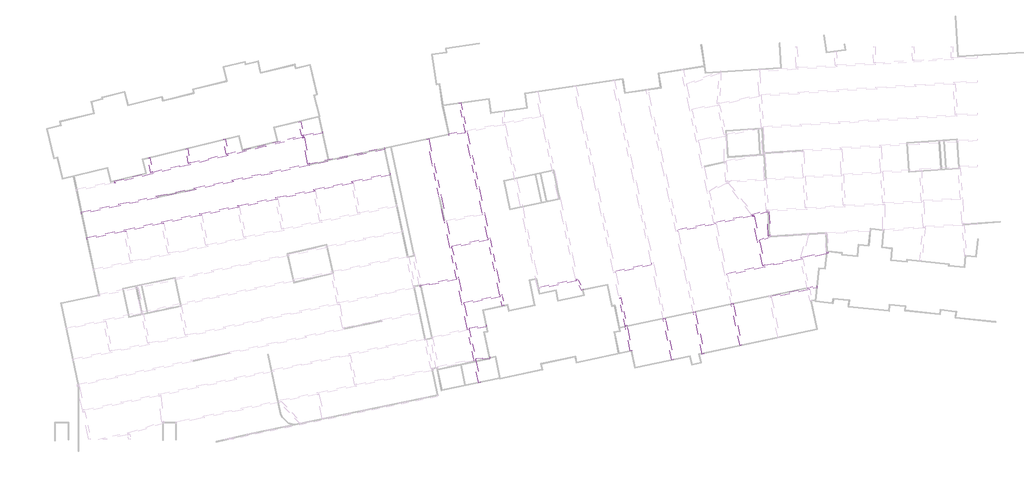
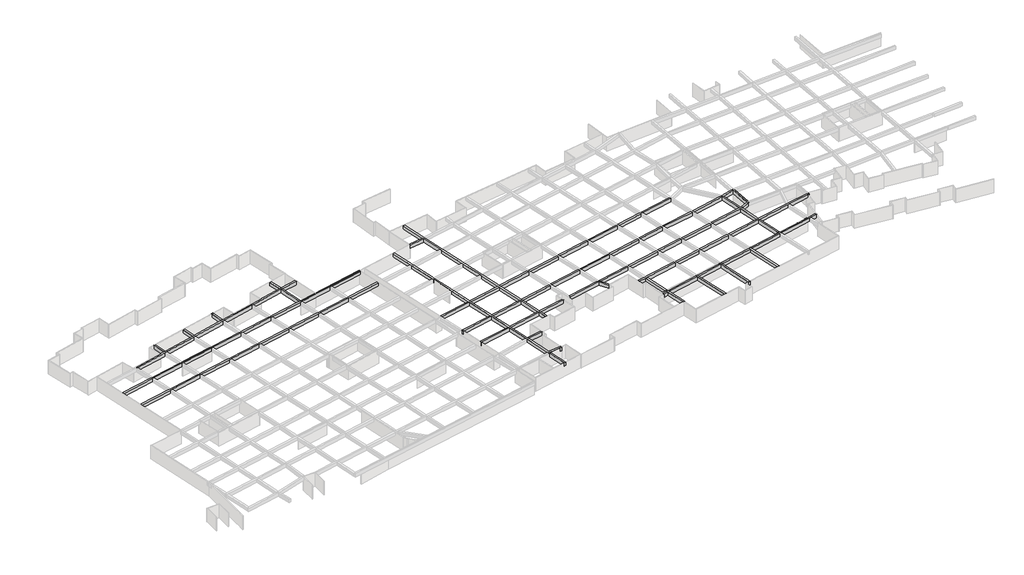
# One storey, part 9 of 14: 33 beams.
"""IFC4 building model written with IfcOpenShell, lengths in millimetres."""

from ifc_helpers import new_model, si_unit, frame, origin, place, context, project, spatial, polyline, outline, extrude, faceted_brep, element, save

model = new_model("IFC4")

# Units and contexts
model_context = context("Model", 3, world=origin())
ifc_project = project(units=[si_unit("LENGTHUNIT", "METRE", prefix="MILLI")], contexts=[model_context])

# Site, building, storey
site = spatial("IfcSite", under=ifc_project)
building = spatial("IfcBuilding", under=site)
storey = spatial("IfcBuildingStorey", under=building, Name="户型图", Elevation=0.0)

# Beams
placement = place(None, origin())
element("IfcBeam", 1, ObjectType="混凝土 - 矩形梁 : KL_beam", at=placement, inside=storey, context=model_context, shape_type="Brep", body=[
    faceted_brep([(-288393.3904984, -144066.4161825, 3300.0), (-303839.5822954, -147811.5548627, 3300.0), (-304228.7284594, -147905.9086277, 3300.0), (-311610.250183, -149695.6586768, 3300.0), (-311999.3963469, -149790.0124418, 3300.0), (-319359.3633104, -151574.5362469, 3300.0), (-319748.5094743, -151668.8900119, 3300.0), (-327267.044724, -153491.8608485, 3300.0), (-327178.3172304, -153881.9374755, 3300.0), (-326986.6349567, -153835.4615086, 3300.0), (-319668.5820962, -152061.1003462, 3300.0), (-319279.6883606, -151966.8077859, 3300.0), (-311919.2779813, -150182.1764686, 3300.0), (-311530.3946325, -150087.8864267, 3300.0), (-304148.8010812, -148298.1189621, 3300.0), (-303759.9073457, -148203.8264018, 3300.0), (-296335.6153384, -146403.7061174, 3300.0), (-295946.7216029, -146309.4135571, 3300.0), (-288504.0259967, -144504.8310706, 3300.0), (-288304.6630048, -144456.4928095, 3300.0), (-327178.3172304, -153881.9374755, 2500.0), (-326986.6349567, -153835.4615086, 2500.0), (-319668.5820962, -152061.1003462, 2500.0), (-319279.6883606, -151966.8077859, 2500.0), (-311919.2779813, -150182.1764686, 2500.0), (-311530.3946325, -150087.8864267, 2500.0), (-304148.8010812, -148298.1189621, 2500.0), (-303759.9073457, -148203.8264018, 2500.0), (-296335.6153384, -146403.7061174, 2500.0), (-295946.7216029, -146309.4135571, 2500.0), (-288504.0259967, -144504.8310706, 2500.0), (-288304.6630048, -144456.4928095, 2500.0), (-327267.044724, -153491.8608485, 2500.0), (-319748.5094743, -151668.8900119, 2500.0), (-319359.3633104, -151574.5362469, 2500.0), (-311999.3963469, -149790.0124418, 2500.0), (-311610.250183, -149695.6586768, 2500.0), (-304228.7284594, -147905.9086277, 2500.0), (-303839.5822954, -147811.5548627, 2500.0), (-288393.3904984, -144066.4161825, 2500.0)], [[[0, 1, 2, 3, 4, 5, 6, 7, 8, 9, 10, 11, 12, 13, 14, 15, 16, 17, 18, 19]], [[19, 18, 17, 16, 15, 14, 13, 12, 11, 10, 9, 8, 20, 21, 22, 23, 24, 25, 26, 27, 28, 29, 30, 31]], [[31, 30, 29, 28, 27, 26, 25, 24, 23, 22, 21, 20, 32, 33, 34, 35, 36, 37, 38, 39]], [[7, 6, 5, 4, 3, 2, 1, 0, 39, 38, 37, 36, 35, 34, 33, 32]], [[7, 32, 20, 8]], [[0, 19, 31, 39]]]),
])
element("IfcBeam", 2, ObjectType="混凝土 - 矩形梁 : KL_beam", at=placement, inside=storey, context=model_context, shape_type="Brep", body=[
    faceted_brep([(-284402.4891232, -143218.1239082, 3300.0), (-284319.3244469, -143609.3829485, 3300.0), (-284319.3244469, -143609.3829485, 2500.0), (-284402.4891232, -143218.1239082, 2500.0), (-288200.5117757, -144025.4185444, 3300.0), (-288393.3904984, -144066.4161825, 3300.0), (-288304.6630048, -144456.4928095, 3300.0), (-288113.8961147, -144415.9440553, 3300.0), (-288304.6630048, -144456.4928095, 2500.0), (-288113.8961147, -144415.9440553, 2500.0), (-288393.3904984, -144066.4161825, 2500.0), (-288200.5117757, -144025.4185444, 2500.0)], [[[0, 1, 2, 3]], [[1, 0, 4, 5, 6, 7]], [[2, 1, 7, 6, 8, 9]], [[3, 2, 9, 8, 10, 11]], [[0, 3, 11, 10, 5, 4]], [[5, 10, 8, 6]]]),
])
element("IfcBeam", 3, ObjectType="混凝土 - 矩形梁 : KL_beam", at=placement, inside=storey, context=model_context, shape_type="SweptSolid", body=[
    extrude(outline(polyline([(-289274.6055614, -141296.103949), (-288885.8925062, -141201.7526868), (-288200.5117757, -144025.4185444), (-288393.3904984, -144066.4161825), (-288590.5706614, -144114.2251872), (-289274.6055614, -141296.103949)])), frame((0.0, 0.0, 2500.0), z_axis=(0.0, 0.0, 1.0), x_axis=(1.0, 0.0, 0.0)), (0.0, 0.0, 1.0), 800.0),
])
element("IfcBeam", 4, ObjectType="混凝土 - 矩形梁 : KL_beam", at=placement, inside=storey, context=model_context, shape_type="SweptSolid", body=[
    extrude(outline(polyline([(-304823.3719195, -144846.7332269), (-304430.7210461, -144770.4096288), (-303839.5822954, -147811.5548627), (-304228.7284594, -147905.9086277), (-304823.3719195, -144846.7332269)])), frame((0.0, 0.0, 2500.0), z_axis=(0.0, 0.0, 1.0), x_axis=(1.0, 0.0, 0.0)), (0.0, 0.0, 1.0), 800.0),
])
element("IfcBeam", 5, ObjectType="混凝土 - 矩形梁 : KL_beam", at=placement, inside=storey, context=model_context, shape_type="SweptSolid", body=[
    extrude(outline(polyline([(-312574.5677396, -146831.0121441), (-312181.9168662, -146754.6885459), (-311610.250183, -149695.6586768), (-311999.3963469, -149790.0124418), (-312574.5677396, -146831.0121441)])), frame((0.0, 0.0, 2500.0), z_axis=(0.0, 0.0, 1.0), x_axis=(1.0, 0.0, 0.0)), (0.0, 0.0, 1.0), 800.0),
])
element("IfcBeam", 6, ObjectType="混凝土 - 矩形梁 : KL_beam", at=placement, inside=storey, context=model_context, shape_type="SweptSolid", body=[
    extrude(outline(polyline([(-320323.3003914, -148711.8470911), (-319930.649518, -148635.523493), (-319359.3633104, -151574.5362469), (-319748.5094743, -151668.8900119), (-320323.3003914, -148711.8470911)])), frame((0.0, 0.0, 2500.0), z_axis=(0.0, 0.0, 1.0), x_axis=(1.0, 0.0, 0.0)), (0.0, 0.0, 1.0), 800.0),
])
element("IfcBeam", 7, ObjectType="混凝土 - 矩形梁 : KL_beam", at=placement, inside=storey, context=model_context, shape_type="Brep", body=[
    faceted_brep([(-271576.7058607, -146561.7487568, 3300.0), (-271493.5411843, -146953.0077971, 3300.0), (-271493.5411843, -146953.0077971, 2500.0), (-271576.7058607, -146561.7487568, 2500.0), (-334091.0971712, -159849.5928286, 3300.0), (-334091.0971712, -159849.5928286, 2500.0), (-334007.9324948, -160240.8518689, 2500.0), (-334007.9324948, -160240.8518689, 3300.0), (-287020.5801813, -149844.4455812, 3300.0), (-287411.8616009, -149927.6150144, 3300.0), (-294841.9553377, -151506.930192, 3300.0), (-295233.214378, -151590.0948684, 3300.0), (-302702.6619422, -153177.7749602, 3300.0), (-303093.9209824, -153260.9396365, 3300.0), (-310515.8719459, -154838.5240142, 3300.0), (-310907.1311647, -154921.6887284, 3300.0), (-318316.8363826, -156496.6701926, 3300.0), (-318708.0954229, -156579.8348689, 3300.0), (-326070.6576793, -158144.7957872, 3300.0), (-326461.9167196, -158227.9604635, 3300.0), (-326378.7520433, -158619.2195038, 3300.0), (-325987.493003, -158536.0548275, 3300.0), (-318624.9307466, -156971.0939092, 3300.0), (-318233.6717063, -156887.9292328, 3300.0), (-310823.5927811, -155312.8683348, 3300.0), (-310432.3335623, -155229.7036205, 3300.0), (-303010.7563061, -153652.1986768, 3300.0), (-302619.4972658, -153569.0340005, 3300.0), (-295150.0497017, -151981.3539087, 3300.0), (-294758.7906614, -151898.1892323, 3300.0), (-287331.8776756, -150319.5501442, 3300.0), (-286940.6186353, -150236.3854679, 3300.0), (-279504.6810453, -148655.828141, 3300.0), (-279113.422005, -148572.6634647, 3300.0), (-326378.7520433, -158619.2195038, 2500.0), (-325987.493003, -158536.0548275, 2500.0), (-318624.9307466, -156971.0939092, 2500.0), (-318233.6717063, -156887.9292328, 2500.0), (-310823.5927811, -155312.8683348, 2500.0), (-310432.3335623, -155229.7036205, 2500.0), (-303010.7563061, -153652.1986768, 2500.0), (-302619.4972658, -153569.0340005, 2500.0), (-295150.0497017, -151981.3539087, 2500.0), (-294758.7906614, -151898.1892323, 2500.0), (-287331.8776756, -150319.5501442, 2500.0), (-286940.6186353, -150236.3854679, 2500.0), (-279504.6810453, -148655.828141, 2500.0), (-279113.422005, -148572.6634647, 2500.0), (-326461.9167196, -158227.9604635, 2500.0), (-326070.6576793, -158144.7957872, 2500.0), (-318708.0954229, -156579.8348689, 2500.0), (-318316.8363826, -156496.6701926, 2500.0), (-310907.1311647, -154921.6887284, 2500.0), (-310515.8719459, -154838.5240142, 2500.0), (-303093.9209824, -153260.9396365, 2500.0), (-302702.6619422, -153177.7749602, 2500.0), (-295233.214378, -151590.0948684, 2500.0), (-294841.9553377, -151506.930192, 2500.0), (-287411.8616009, -149927.6150144, 2500.0), (-287020.5801813, -149844.4455812, 2500.0)], [[[0, 1, 2, 3]], [[4, 5, 6, 7]], [[1, 0, 8, 9, 10, 11, 12, 13, 14, 15, 16, 17, 18, 19, 4, 7, 20, 21, 22, 23, 24, 25, 26, 27, 28, 29, 30, 31, 32, 33]], [[2, 1, 33, 32, 31, 30, 29, 28, 27, 26, 25, 24, 23, 22, 21, 20, 7, 6, 34, 35, 36, 37, 38, 39, 40, 41, 42, 43, 44, 45, 46, 47]], [[3, 2, 47, 46, 45, 44, 43, 42, 41, 40, 39, 38, 37, 36, 35, 34, 6, 5, 48, 49, 50, 51, 52, 53, 54, 55, 56, 57, 58, 59]], [[0, 3, 59, 58, 57, 56, 55, 54, 53, 52, 51, 50, 49, 48, 5, 4, 19, 18, 17, 16, 15, 14, 13, 12, 11, 10, 9, 8]]]),
])
element("IfcBeam", 8, ObjectType="混凝土 - 矩形梁 : KL_beam", at=placement, inside=storey, context=model_context, shape_type="Brep", body=[
    faceted_brep([(-270449.8244964, -151863.3087528, 3300.0), (-270366.6598201, -152254.5677931, 3300.0), (-270366.6598201, -152254.5677931, 2500.0), (-270449.8244964, -151863.3087528, 2500.0), (-332964.2158069, -165151.1528246, 3300.0), (-332964.2158069, -165151.1528246, 2500.0), (-332881.0511306, -165542.4118649, 2500.0), (-332881.0511306, -165542.4118649, 3300.0), (-278069.7053171, -153482.9644203, 3300.0), (-278460.9643574, -153566.1290967, 3300.0), (-285896.9019474, -155146.6864236, 3300.0), (-286288.1609877, -155229.8510999, 3300.0), (-293715.0739735, -156808.490188, 3300.0), (-294106.3330138, -156891.6548643, 3300.0), (-301575.7805779, -158479.3349561, 3300.0), (-301967.0396182, -158562.4996325, 3300.0), (-309383.926848, -160139.0076803, 3300.0), (-309775.1860668, -160222.1723946, 3300.0), (-317189.9550184, -161798.2301885, 3300.0), (-317581.2140587, -161881.3948649, 3300.0), (-324943.7763151, -163446.3557832, 3300.0), (-325335.0353554, -163529.5204595, 3300.0), (-325251.870679, -163920.7794998, 3300.0), (-324860.6116388, -163837.6148234, 3300.0), (-317498.0493824, -162272.6539051, 3300.0), (-317106.7903421, -162189.4892288, 3300.0), (-309691.6476832, -160613.3520009, 3300.0), (-309300.3884644, -160530.1872867, 3300.0), (-301883.8749419, -158953.7586728, 3300.0), (-301492.6159016, -158870.5939964, 3300.0), (-294023.1683375, -157282.9139046, 3300.0), (-293631.9092972, -157199.7492283, 3300.0), (-286204.9963114, -155621.1101402, 3300.0), (-285813.7372711, -155537.9454639, 3300.0), (-278377.799681, -153957.388137, 3300.0), (-277986.5406407, -153874.2234606, 3300.0), (-325251.870679, -163920.7794998, 2500.0), (-324860.6116388, -163837.6148234, 2500.0), (-317498.0493824, -162272.6539051, 2500.0), (-317106.7903421, -162189.4892288, 2500.0), (-309691.6476832, -160613.3520009, 2500.0), (-309300.3884644, -160530.1872867, 2500.0), (-301883.8749419, -158953.7586728, 2500.0), (-301492.6159016, -158870.5939964, 2500.0), (-294023.1683375, -157282.9139046, 2500.0), (-293631.9092972, -157199.7492283, 2500.0), (-286204.9963114, -155621.1101402, 2500.0), (-285813.7372711, -155537.9454639, 2500.0), (-278377.799681, -153957.388137, 2500.0), (-277986.5406407, -153874.2234606, 2500.0), (-325335.0353554, -163529.5204595, 2500.0), (-324943.7763151, -163446.3557832, 2500.0), (-317581.2140587, -161881.3948649, 2500.0), (-317189.9550184, -161798.2301885, 2500.0), (-309775.1860668, -160222.1723946, 2500.0), (-309383.926848, -160139.0076803, 2500.0), (-301967.0396182, -158562.4996325, 2500.0), (-301575.7805779, -158479.3349561, 2500.0), (-294106.3330138, -156891.6548643, 2500.0), (-293715.0739735, -156808.490188, 2500.0), (-286288.1609877, -155229.8510999, 2500.0), (-285896.9019474, -155146.6864236, 2500.0), (-278460.9643574, -153566.1290967, 2500.0), (-278069.7053171, -153482.9644203, 2500.0)], [[[0, 1, 2, 3]], [[4, 5, 6, 7]], [[1, 0, 8, 9, 10, 11, 12, 13, 14, 15, 16, 17, 18, 19, 20, 21, 4, 7, 22, 23, 24, 25, 26, 27, 28, 29, 30, 31, 32, 33, 34, 35]], [[2, 1, 35, 34, 33, 32, 31, 30, 29, 28, 27, 26, 25, 24, 23, 22, 7, 6, 36, 37, 38, 39, 40, 41, 42, 43, 44, 45, 46, 47, 48, 49]], [[3, 2, 49, 48, 47, 46, 45, 44, 43, 42, 41, 40, 39, 38, 37, 36, 6, 5, 50, 51, 52, 53, 54, 55, 56, 57, 58, 59, 60, 61, 62, 63]], [[0, 3, 63, 62, 61, 60, 59, 58, 57, 56, 55, 54, 53, 52, 51, 50, 5, 4, 21, 20, 19, 18, 17, 16, 15, 14, 13, 12, 11, 10, 9, 8]]]),
])
element("IfcBeam", 9, ObjectType="混凝土 - 矩形梁 : KL_beam", at=placement, inside=storey, context=model_context, shape_type="SweptSolid", body=[
    extrude(outline(polyline([(-288504.0259967, -144504.8310706), (-288304.6630048, -144456.4928095), (-288113.8961147, -144415.9440553), (-287020.5801813, -149844.4455812), (-287411.8616009, -149927.6150144), (-288504.0259967, -144504.8310706)])), frame((0.0, 0.0, 2500.0), z_axis=(0.0, 0.0, 1.0), x_axis=(1.0, 0.0, 0.0)), (0.0, 0.0, 1.0), 800.0),
])
element("IfcBeam", 10, ObjectType="混凝土 - 矩形梁 : KL_beam", at=placement, inside=storey, context=model_context, shape_type="Brep", body=[
    faceted_brep([(-251742.5078886, -195066.5259973, 3300.0), (-252133.7669289, -195149.6906737, 3300.0), (-252133.7669289, -195149.6906737, 2500.0), (-251742.5078886, -195066.5259973, 2500.0), (-262438.9406461, -144743.7663824, 3300.0), (-262438.9406461, -144743.7663824, 2500.0), (-262830.1996864, -144826.9310587, 2500.0), (-262830.1996864, -144826.9310587, 3300.0), (-252718.5927921, -190474.4075708, 3300.0), (-252802.1941039, -190081.0943222, 3300.0), (-254061.3718629, -184157.1287242, 3300.0), (-254144.5872317, -183765.6311942, 3300.0), (-255169.8458295, -178942.168725, 3300.0), (-255253.0105059, -178550.9096847, 3300.0), (-256292.2110421, -173661.8555521, 3300.0), (-256375.3764788, -173270.5929347, 3300.0), (-257657.9882479, -167236.3789868, 3300.0), (-257741.1529242, -166845.1199465, 3300.0), (-258766.7490607, -162020.0694828, 3300.0), (-258849.913737, -161628.8104425, 3300.0), (-259903.4345087, -156672.3848989, 3300.0), (-259986.5991851, -156281.1258586, 3300.0), (-261262.1742572, -150280.0169676, 3300.0), (-261345.3389335, -149888.7579273, 3300.0), (-261736.5979738, -149971.9226036, 3300.0), (-261653.4332975, -150363.1816439, 3300.0), (-260377.8582254, -156364.2905349, 3300.0), (-260294.693549, -156755.5495752, 3300.0), (-259241.1727773, -161711.9751188, 3300.0), (-259158.008101, -162103.2341591, 3300.0), (-258132.4119645, -166928.2846229, 3300.0), (-258049.2472882, -167319.5436632, 3300.0), (-256766.2798961, -173355.4306854, 3300.0), (-256683.1144595, -173746.6933028, 3300.0), (-255644.2695462, -178634.074361, 3300.0), (-255561.1048698, -179025.3334013, 3300.0), (-254535.8170874, -183848.9331735, 3300.0), (-254452.599585, -184240.4407408, 3300.0), (-253197.5014394, -190145.2132669, 3300.0), (-253114.3367631, -190536.4723072, 3300.0), (-261736.5979738, -149971.9226036, 2500.0), (-261653.4332975, -150363.1816439, 2500.0), (-260377.8582254, -156364.2905349, 2500.0), (-260294.693549, -156755.5495752, 2500.0), (-259241.1727773, -161711.9751188, 2500.0), (-259158.008101, -162103.2341591, 2500.0), (-258132.4119645, -166928.2846229, 2500.0), (-258049.2472882, -167319.5436632, 2500.0), (-256766.2798961, -173355.4306854, 2500.0), (-256683.1144595, -173746.6933028, 2500.0), (-255644.2695462, -178634.074361, 2500.0), (-255561.1048698, -179025.3334013, 2500.0), (-254535.8170874, -183848.9331735, 2500.0), (-254452.599585, -184240.4407408, 2500.0), (-253197.5014394, -190145.2132669, 2500.0), (-253114.3367631, -190536.4723072, 2500.0), (-261345.3389335, -149888.7579273, 2500.0), (-261262.1742572, -150280.0169676, 2500.0), (-259986.5991851, -156281.1258586, 2500.0), (-259903.4345087, -156672.3848989, 2500.0), (-258849.913737, -161628.8104425, 2500.0), (-258766.7490607, -162020.0694828, 2500.0), (-257741.1529242, -166845.1199465, 2500.0), (-257657.9882479, -167236.3789868, 2500.0), (-256375.3764788, -173270.5929347, 2500.0), (-256292.2110421, -173661.8555521, 2500.0), (-255253.0105059, -178550.9096847, 2500.0), (-255169.8458295, -178942.168725, 2500.0), (-254144.5872317, -183765.6311942, 2500.0), (-254061.3718629, -184157.1287242, 2500.0), (-252802.1941039, -190081.0943222, 2500.0), (-252718.5927921, -190474.4075708, 2500.0)], [[[0, 1, 2, 3]], [[4, 5, 6, 7]], [[1, 0, 8, 9, 10, 11, 12, 13, 14, 15, 16, 17, 18, 19, 20, 21, 22, 23, 4, 7, 24, 25, 26, 27, 28, 29, 30, 31, 32, 33, 34, 35, 36, 37, 38, 39]], [[2, 1, 39, 38, 37, 36, 35, 34, 33, 32, 31, 30, 29, 28, 27, 26, 25, 24, 7, 6, 40, 41, 42, 43, 44, 45, 46, 47, 48, 49, 50, 51, 52, 53, 54, 55]], [[3, 2, 55, 54, 53, 52, 51, 50, 49, 48, 47, 46, 45, 44, 43, 42, 41, 40, 6, 5, 56, 57, 58, 59, 60, 61, 62, 63, 64, 65, 66, 67, 68, 69, 70, 71]], [[0, 3, 71, 70, 69, 68, 67, 66, 65, 64, 63, 62, 61, 60, 59, 58, 57, 56, 5, 4, 23, 22, 21, 20, 19, 18, 17, 16, 15, 14, 13, 12, 11, 10, 9, 8]]]),
])
element("IfcBeam", 11, ObjectType="混凝土 - 矩形梁 : KL_beam", at=placement, inside=storey, context=model_context, shape_type="Brep", body=[
    faceted_brep([(-256201.338367, -137355.4226333, 3300.0), (-255810.0793267, -137272.257957, 3300.0), (-255810.0793267, -137272.257957, 2500.0), (-256201.338367, -137355.4226333, 2500.0), (-247302.718, -179220.1399447, 3300.0), (-247302.718, -179220.1399447, 2500.0), (-246911.4589597, -179136.9752684, 2500.0), (-246911.4589597, -179136.9752684, 3300.0), (-254972.9847902, -143134.3718556, 3300.0), (-254889.7059832, -143526.1678387, 3300.0), (-253874.8161124, -148300.8492826, 3300.0), (-253791.6514361, -148692.1083228, 3300.0), (-252516.076364, -154693.2172139, 3300.0), (-252432.9116877, -155084.4762542, 3300.0), (-251379.390916, -160040.9017978, 3300.0), (-251296.2262396, -160432.160838, 3300.0), (-250270.6301032, -165257.2113018, 3300.0), (-250187.4654268, -165648.4703421, 3300.0), (-248911.6437611, -171650.7393651, 3300.0), (-248828.4783244, -172042.0019825, 3300.0), (-247782.4876848, -176963.00104, 3300.0), (-247699.3230085, -177354.2600803, 3300.0), (-247308.0639682, -177271.0954039, 3300.0), (-247391.2286445, -176879.8363636, 3300.0), (-248437.5749071, -171957.1642317, 3300.0), (-248520.7403438, -171565.9016143, 3300.0), (-249796.2063865, -165565.3056658, 3300.0), (-249879.3710629, -165174.0466255, 3300.0), (-250904.9671993, -160348.9961617, 3300.0), (-250988.1318757, -159957.7371214, 3300.0), (-252041.6526474, -155001.3115779, 3300.0), (-252124.8173237, -154610.0525376, 3300.0), (-253400.3923958, -148608.9436465, 3300.0), (-253483.5570721, -148217.6846062, 3300.0), (-254496.3247703, -143452.9871997, 3300.0), (-254579.4894466, -143061.7281594, 3300.0), (-247308.0639682, -177271.0954039, 2500.0), (-247391.2286445, -176879.8363636, 2500.0), (-248437.5749071, -171957.1642317, 2500.0), (-248520.7403438, -171565.9016143, 2500.0), (-249796.2063865, -165565.3056658, 2500.0), (-249879.3710629, -165174.0466255, 2500.0), (-250904.9671993, -160348.9961617, 2500.0), (-250988.1318757, -159957.7371214, 2500.0), (-252041.6526474, -155001.3115779, 2500.0), (-252124.8173237, -154610.0525376, 2500.0), (-253400.3923958, -148608.9436465, 2500.0), (-253483.5570721, -148217.6846062, 2500.0), (-254496.3247703, -143452.9871997, 2500.0), (-254579.4894466, -143061.7281594, 2500.0), (-247699.3230085, -177354.2600803, 2500.0), (-247782.4876848, -176963.00104, 2500.0), (-248828.4783244, -172042.0019825, 2500.0), (-248911.6437611, -171650.7393651, 2500.0), (-250187.4654268, -165648.4703421, 2500.0), (-250270.6301032, -165257.2113018, 2500.0), (-251296.2262396, -160432.160838, 2500.0), (-251379.390916, -160040.9017978, 2500.0), (-252432.9116877, -155084.4762542, 2500.0), (-252516.076364, -154693.2172139, 2500.0), (-253791.6514361, -148692.1083228, 2500.0), (-253874.8161124, -148300.8492826, 2500.0), (-254889.7059832, -143526.1678387, 2500.0), (-254972.9847902, -143134.3718556, 2500.0)], [[[0, 1, 2, 3]], [[4, 5, 6, 7]], [[1, 0, 8, 9, 10, 11, 12, 13, 14, 15, 16, 17, 18, 19, 20, 21, 4, 7, 22, 23, 24, 25, 26, 27, 28, 29, 30, 31, 32, 33, 34, 35]], [[2, 1, 35, 34, 33, 32, 31, 30, 29, 28, 27, 26, 25, 24, 23, 22, 7, 6, 36, 37, 38, 39, 40, 41, 42, 43, 44, 45, 46, 47, 48, 49]], [[3, 2, 49, 48, 47, 46, 45, 44, 43, 42, 41, 40, 39, 38, 37, 36, 6, 5, 50, 51, 52, 53, 54, 55, 56, 57, 58, 59, 60, 61, 62, 63]], [[0, 3, 63, 62, 61, 60, 59, 58, 57, 56, 55, 54, 53, 52, 51, 50, 5, 4, 21, 20, 19, 18, 17, 16, 15, 14, 13, 12, 11, 10, 9, 8]]]),
])
element("IfcBeam", 12, ObjectType="混凝土 - 矩形梁 : KL_beam", at=placement, inside=storey, context=model_context, shape_type="Brep", body=[
    faceted_brep([(-230526.1919186, -175828.6497309, 3300.0), (-230871.4825432, -176030.5764121, 3300.0), (-230871.4825432, -176030.5764121, 2500.0), (-230526.1919186, -175828.6497309, 2500.0), (-231587.5550809, -174013.7397486, 3300.0), (-231776.7079802, -173690.2920379, 3300.0), (-232154.5574648, -173836.5437133, 3300.0), (-231999.7015891, -174101.3441932, 3300.0), (-232154.5574648, -173836.5437133, 2500.0), (-231999.7015891, -174101.3441932, 2500.0), (-231776.7079802, -173690.2920379, 2500.0), (-231587.5550809, -174013.7397486, 2500.0)], [[[0, 1, 2, 3]], [[1, 0, 4, 5, 6, 7]], [[2, 1, 7, 6, 8, 9]], [[3, 2, 9, 8, 10, 11]], [[0, 3, 11, 10, 5, 4]], [[5, 10, 8, 6]]]),
])
element("IfcBeam", 13, ObjectType="混凝土 - 矩形梁 : KL_beam", at=placement, inside=storey, context=model_context, shape_type="SweptSolid", body=[
    extrude(outline(polyline([(-221980.5936609, -183397.2342456), (-223207.2135078, -177626.4415809), (-222815.9544675, -177543.2769046), (-221589.3346206, -183314.0695693), (-221980.5936609, -183397.2342456)])), frame((0.0, 0.0, 2500.0), z_axis=(0.0, 0.0, 1.0), x_axis=(1.0, 0.0, 0.0)), (0.0, 0.0, 1.0), 800.0),
])
element("IfcBeam", 14, ObjectType="混凝土 - 矩形梁 : KL_beam", at=placement, inside=storey, context=model_context, shape_type="SweptSolid", body=[
    extrude(outline(polyline([(-258266.0962037, -144060.9355141), (-258328.6699897, -143665.8601778), (-254972.9847902, -143134.3718556), (-254889.7059832, -143526.1678387), (-258266.0962037, -144060.9355141)])), frame((0.0, 0.0, 2500.0), z_axis=(0.0, 0.0, 1.0), x_axis=(1.0, 0.0, 0.0)), (0.0, 0.0, 1.0), 800.0),
])
element("IfcBeam", 15, ObjectType="混凝土 - 矩形梁 : KL_beam", at=placement, inside=storey, context=model_context, shape_type="SweptSolid", body=[
    extrude(outline(polyline([(-265303.074266, -168861.3921845), (-265386.2389423, -168470.1331442), (-258132.4119645, -166928.2846229), (-258049.2472882, -167319.5436632), (-265303.074266, -168861.3921845)])), frame((0.0, 0.0, 2500.0), z_axis=(0.0, 0.0, 1.0), x_axis=(1.0, 0.0, 0.0)), (0.0, 0.0, 1.0), 800.0),
    extrude(outline(polyline([(-257657.9882479, -167236.3789868), (-257741.1529242, -166845.1199465), (-250270.6301032, -165257.2113018), (-250187.4654268, -165648.4703421), (-257657.9882479, -167236.3789868)])), frame((0.0, 0.0, 2500.0), z_axis=(0.0, 0.0, 1.0), x_axis=(1.0, 0.0, 0.0)), (0.0, 0.0, 1.0), 800.0),
    extrude(outline(polyline([(-249796.2063865, -165565.3056658), (-249879.3710629, -165174.0466255), (-242482.2442457, -163601.738783), (-242399.0795694, -163992.9978233), (-249796.2063865, -165565.3056658)])), frame((0.0, 0.0, 2500.0), z_axis=(0.0, 0.0, 1.0), x_axis=(1.0, 0.0, 0.0)), (0.0, 0.0, 1.0), 800.0),
    extrude(outline(polyline([(-242007.8205291, -163909.833147), (-242090.9852054, -163518.5741067), (-234682.4302819, -161943.8371452), (-234599.2656056, -162335.0961855), (-242007.8205291, -163909.833147)])), frame((0.0, 0.0, 2500.0), z_axis=(0.0, 0.0, 1.0), x_axis=(1.0, 0.0, 0.0)), (0.0, 0.0, 1.0), 800.0),
    extrude(outline(polyline([(-234208.0065653, -162251.9315092), (-234291.1712416, -161860.6724689), (-226892.6007566, -160288.0577653), (-226809.4360803, -160679.3168056), (-234208.0065653, -162251.9315092)])), frame((0.0, 0.0, 2500.0), z_axis=(0.0, 0.0, 1.0), x_axis=(1.0, 0.0, 0.0)), (0.0, 0.0, 1.0), 800.0),
    extrude(outline(polyline([(-226418.17704, -160596.1521293), (-226501.3417163, -160204.893089), (-219067.4199507, -158624.7642388), (-218984.2552744, -159016.023279), (-226418.17704, -160596.1521293)])), frame((0.0, 0.0, 2500.0), z_axis=(0.0, 0.0, 1.0), x_axis=(1.0, 0.0, 0.0)), (0.0, 0.0, 1.0), 800.0),
    extrude(outline(polyline([(-218592.9962341, -158932.8586027), (-218676.1609104, -158541.5995624), (-212821.0159926, -157297.0500906), (-212737.8513162, -157688.3091309), (-218592.9962341, -158932.8586027)])), frame((0.0, 0.0, 2500.0), z_axis=(0.0, 0.0, 1.0), x_axis=(1.0, 0.0, 0.0)), (0.0, 0.0, 1.0), 800.0),
    extrude(outline(polyline([(-212346.5922759, -157605.1444546), (-212429.7569523, -157213.8854143), (-205021.5093866, -155639.2137837), (-204938.3447103, -156030.472824), (-212346.5922759, -157605.1444546)])), frame((0.0, 0.0, 2500.0), z_axis=(0.0, 0.0, 1.0), x_axis=(1.0, 0.0, 0.0)), (0.0, 0.0, 1.0), 800.0),
])
element("IfcBeam", 16, ObjectType="混凝土 - 矩形梁 : KL_beam", at=placement, inside=storey, context=model_context, shape_type="SweptSolid", body=[
    extrude(outline(polyline([(-264167.3475284, -175370.9960627), (-264252.1845035, -174980.0962192), (-256766.2798961, -173355.4306854), (-256683.1144595, -173746.6933028), (-264167.3475284, -175370.9960627)])), frame((0.0, 0.0, 2500.0), z_axis=(0.0, 0.0, 1.0), x_axis=(1.0, 0.0, 0.0)), (0.0, 0.0, 1.0), 800.0),
    extrude(outline(polyline([(-217262.7259588, -165191.2881935), (-217345.8913955, -164800.0255761), (-211496.0683326, -163530.4387449), (-211412.902896, -163921.7013623), (-217262.7259588, -165191.2881935)])), frame((0.0, 0.0, 2500.0), z_axis=(0.0, 0.0, 1.0), x_axis=(1.0, 0.0, 0.0)), (0.0, 0.0, 1.0), 800.0),
    extrude(outline(polyline([(-256292.2110421, -173661.8555521), (-256375.3764788, -173270.5929347), (-248911.6437611, -171650.7393651), (-248828.4783244, -172042.0019825), (-256292.2110421, -173661.8555521)])), frame((0.0, 0.0, 2500.0), z_axis=(0.0, 0.0, 1.0), x_axis=(1.0, 0.0, 0.0)), (0.0, 0.0, 1.0), 800.0),
    extrude(outline(polyline([(-248437.5749071, -171957.1642317), (-248520.7403438, -171565.9016143), (-241130.3369189, -169961.9626978), (-241047.1714822, -170353.2253152), (-248437.5749071, -171957.1642317)])), frame((0.0, 0.0, 2500.0), z_axis=(0.0, 0.0, 1.0), x_axis=(1.0, 0.0, 0.0)), (0.0, 0.0, 1.0), 800.0),
    extrude(outline(polyline([(-240656.2680649, -170268.3875645), (-240739.4335016, -169877.124947), (-233337.6123577, -168270.7080435), (-233254.446921, -168661.9706609), (-240656.2680649, -170268.3875645)])), frame((0.0, 0.0, 2500.0), z_axis=(0.0, 0.0, 1.0), x_axis=(1.0, 0.0, 0.0)), (0.0, 0.0, 1.0), 800.0),
    extrude(outline(polyline([(-232863.5435036, -168577.1329101), (-232946.7089403, -168185.8702927), (-225554.8631598, -166581.6183418), (-225471.6977231, -166972.8809592), (-232863.5435036, -168577.1329101)])), frame((0.0, 0.0, 2500.0), z_axis=(0.0, 0.0, 1.0), x_axis=(1.0, 0.0, 0.0)), (0.0, 0.0, 1.0), 800.0),
    extrude(outline(polyline([(-225080.7943058, -166888.0432085), (-225163.9597425, -166496.7805911), (-217736.7948129, -164884.8633268), (-217653.6293762, -165276.1259443), (-225080.7943058, -166888.0432085)])), frame((0.0, 0.0, 2500.0), z_axis=(0.0, 0.0, 1.0), x_axis=(1.0, 0.0, 0.0)), (0.0, 0.0, 1.0), 800.0),
])
element("IfcBeam", 17, ObjectType="混凝土 - 矩形梁 : KL_beam", at=placement, inside=storey, context=model_context, shape_type="SweptSolid", body=[
    extrude(outline(polyline([(-211021.0898908, -163841.1428861), (-211104.2672354, -163449.824246), (-203668.5336742, -162004.4640578), (-203585.3563296, -162395.7826978), (-211021.0898908, -163841.1428861)])), frame((0.0, 0.0, 2500.0), z_axis=(0.0, 0.0, 1.0), x_axis=(1.0, 0.0, 0.0)), (0.0, 0.0, 1.0), 800.0),
])
element("IfcBeam", 18, ObjectType="混凝土 - 矩形梁 : KL_beam", at=placement, inside=storey, context=model_context, shape_type="Brep", body=[
    faceted_brep([(-195557.0636717, -160692.8542724, 3300.0), (-195653.7540352, -160304.4702057, 3300.0), (-195963.1553621, -160370.2354879, 3300.0), (-203276.5424774, -161924.7439073, 3300.0), (-203193.377801, -162316.0029476, 3300.0), (-195759.4562247, -160735.8741376, 3300.0), (-195557.0636717, -160692.8542724, 2500.0), (-203193.377801, -162316.0029476, 2500.0), (-195759.4562247, -160735.8741376, 2500.0), (-195653.7540352, -160304.4702057, 2500.0), (-203276.5424774, -161924.7439073, 2500.0), (-195963.1553621, -160370.2354879, 2500.0)], [[[0, 1, 2, 3, 4, 5]], [[6, 0, 5, 4, 7, 8]], [[9, 6, 8, 7, 10, 11]], [[1, 9, 11, 10, 3, 2]], [[4, 3, 10, 7]], [[1, 0, 6, 9]]]),
])
element("IfcBeam", 19, ObjectType="混凝土 - 矩形梁 : KL_beam", at=placement, inside=storey, context=model_context, shape_type="Brep", body=[
    faceted_brep([(-192560.4754291, -159419.8343743, 3300.0), (-192847.1376854, -159501.8159013, 3300.0), (-195532.0262334, -160269.6577012, 3300.0), (-195653.7540352, -160304.4702057, 3300.0), (-195557.0636717, -160692.8542724, 3300.0), (-195370.9760893, -160639.6357415, 3300.0), (-192710.6636864, -159878.8223865, 3300.0), (-192492.3575326, -159816.3897801, 3300.0), (-195557.0636717, -160692.8542724, 2500.0), (-195370.9760893, -160639.6357415, 2500.0), (-192710.6636864, -159878.8223865, 2500.0), (-192492.3575326, -159816.3897801, 2500.0), (-195653.7540352, -160304.4702057, 2500.0), (-195532.0262334, -160269.6577012, 2500.0), (-192847.1376854, -159501.8159013, 2500.0), (-192560.4754291, -159419.8343743, 2500.0)], [[[0, 1, 2, 3, 4, 5, 6, 7]], [[7, 6, 5, 4, 8, 9, 10, 11]], [[11, 10, 9, 8, 12, 13, 14, 15]], [[3, 2, 1, 0, 15, 14, 13, 12]], [[3, 12, 8, 4]], [[0, 7, 11, 15]]]),
])
element("IfcBeam", 20, ObjectType="混凝土 - 矩形梁 : KL_beam", at=placement, inside=storey, context=model_context, shape_type="SweptSolid", body=[
    extrude(outline(polyline([(-241350.8096735, -175595.9056761), (-241267.6449972, -175987.1647164), (-247308.0639682, -177271.0954039), (-247391.2286445, -176879.8363636), (-241350.8096735, -175595.9056761)])), frame((0.0, 0.0, 2500.0), z_axis=(0.0, 0.0, 1.0), x_axis=(1.0, 0.0, 0.0)), (0.0, 0.0, 1.0), 800.0),
    extrude(outline(polyline([(-262928.7236154, -180591.3691096), (-263011.8882918, -180200.1100693), (-255644.2695462, -178634.074361), (-255561.1048698, -179025.3334013), (-262928.7236154, -180591.3691096)])), frame((0.0, 0.0, 2500.0), z_axis=(0.0, 0.0, 1.0), x_axis=(1.0, 0.0, 0.0)), (0.0, 0.0, 1.0), 800.0),
    extrude(outline(polyline([(-255169.8458295, -178942.168725), (-255253.0105059, -178550.9096847), (-247782.4876848, -176963.00104), (-247699.3230085, -177354.2600803), (-255169.8458295, -178942.168725)])), frame((0.0, 0.0, 2500.0), z_axis=(0.0, 0.0, 1.0), x_axis=(1.0, 0.0, 0.0)), (0.0, 0.0, 1.0), 800.0),
])
element("IfcBeam", 21, ObjectType="混凝土 - 矩形梁 : KL_beam", at=placement, inside=storey, context=model_context, shape_type="SweptSolid", body=[
    extrude(outline(polyline([(-250609.9684126, -183142.3825299), (-250540.5091415, -183536.3056311), (-254061.3718629, -184157.1287242), (-254144.5872317, -183765.6311942), (-250609.9684126, -183142.3825299)])), frame((0.0, 0.0, 2500.0), z_axis=(0.0, 0.0, 1.0), x_axis=(1.0, 0.0, 0.0)), (0.0, 0.0, 1.0), 800.0),
])
element("IfcBeam", 22, ObjectType="混凝土 - 矩形梁 : KL_beam", at=placement, inside=storey, context=model_context, shape_type="SweptSolid", body=[
    extrude(outline(polyline([(-239502.5663622, -175696.1273321), (-239585.7310386, -175304.8682918), (-232177.1761151, -173730.1313303), (-232154.5574648, -173836.5437133), (-231999.7015891, -174101.3441932), (-239502.5663622, -175696.1273321)])), frame((0.0, 0.0, 2500.0), z_axis=(0.0, 0.0, 1.0), x_axis=(1.0, 0.0, 0.0)), (0.0, 0.0, 1.0), 800.0),
])
element("IfcBeam", 23, ObjectType="混凝土 - 矩形梁 : KL_beam", at=placement, inside=storey, context=model_context, shape_type="SweptSolid", body=[
    extrude(outline(polyline([(-202041.8315032, -167733.6023328), (-202124.9961795, -167342.3432925), (-194691.0746032, -165762.2144825), (-194607.9099268, -166153.4735228), (-202041.8315032, -167733.6023328)])), frame((0.0, 0.0, 2500.0), z_axis=(0.0, 0.0, 1.0), x_axis=(1.0, 0.0, 0.0)), (0.0, 0.0, 1.0), 800.0),
    extrude(outline(polyline([(-231587.5550809, -174013.7397486), (-231776.7079802, -173690.2920379), (-231785.9170748, -173646.966654), (-224387.3465898, -172074.3519504), (-224304.1819135, -172465.6109907), (-231587.5550809, -174013.7397486)])), frame((0.0, 0.0, 2500.0), z_axis=(0.0, 0.0, 1.0), x_axis=(1.0, 0.0, 0.0)), (0.0, 0.0, 1.0), 800.0),
    extrude(outline(polyline([(-223912.9228732, -172382.4463144), (-223996.0875495, -171991.1872741), (-216562.1657839, -170411.0584239), (-216479.0011076, -170802.3174642), (-223912.9228732, -172382.4463144)])), frame((0.0, 0.0, 2500.0), z_axis=(0.0, 0.0, 1.0), x_axis=(1.0, 0.0, 0.0)), (0.0, 0.0, 1.0), 800.0),
    extrude(outline(polyline([(-216087.7420673, -170719.1527879), (-216170.9067436, -170327.8937476), (-210315.7618257, -169083.3442757), (-210232.5971494, -169474.603316), (-216087.7420673, -170719.1527879)])), frame((0.0, 0.0, 2500.0), z_axis=(0.0, 0.0, 1.0), x_axis=(1.0, 0.0, 0.0)), (0.0, 0.0, 1.0), 800.0),
    extrude(outline(polyline([(-209841.3381091, -169391.4386397), (-209924.5027854, -169000.1795994), (-202516.2552198, -167425.5079689), (-202433.0905435, -167816.7670092), (-209841.3381091, -169391.4386397)])), frame((0.0, 0.0, 2500.0), z_axis=(0.0, 0.0, 1.0), x_axis=(1.0, 0.0, 0.0)), (0.0, 0.0, 1.0), 800.0),
])
element("IfcBeam", 24, ObjectType="混凝土 - 矩形梁 : KL_beam", at=placement, inside=storey, context=model_context, shape_type="Brep", body=[
    faceted_brep([(-194308.9688434, -165635.987007, 3300.0), (-194223.8899677, -166036.2516472, 3300.0), (-192150.3287913, -165105.3594505, 3300.0), (-191990.8566446, -165033.7669754, 3300.0), (-192011.7600695, -164696.0180214, 3300.0), (-192017.2594885, -164607.1606673, 3300.0), (-192407.1907126, -164782.2140671, 3300.0), (-194223.8899677, -166036.2516472, 2500.0), (-192150.3287913, -165105.3594505, 2500.0), (-191990.8566446, -165033.7669754, 2500.0), (-194308.9688434, -165635.987007, 2500.0), (-192407.1907126, -164782.2140671, 2500.0), (-192017.2594885, -164607.1606673, 2500.0), (-192011.7600695, -164696.0180214, 2500.0)], [[[0, 1, 2, 3, 4, 5, 6]], [[1, 7, 8, 9, 3, 2]], [[7, 10, 11, 12, 13, 9, 8]], [[5, 12, 11, 10, 0, 6]], [[0, 10, 7, 1]], [[5, 4, 3, 9, 13, 12]]]),
])
element("IfcBeam", 25, ObjectType="混凝土 - 矩形梁 : KL_beam", at=placement, inside=storey, context=model_context, shape_type="Brep", body=[
    faceted_brep([(-224940.093163, -177585.8402843, 3300.0), (-224940.093163, -177585.8402843, 2500.0), (-224856.9284867, -177977.0993246, 2500.0), (-224856.9284867, -177977.0993246, 3300.0), (-215465.1973783, -175571.8890141, 3300.0), (-215382.032702, -175963.1480544, 3300.0), (-215382.032702, -175963.1480544, 2500.0), (-215465.1973783, -175571.8890141, 2500.0), (-223207.2135078, -177626.4415809, 3300.0), (-222815.9544675, -177543.2769046, 3300.0), (-222899.1191439, -177152.0178643, 3300.0), (-223290.3781842, -177235.1825406, 3300.0), (-223207.2135078, -177626.4415809, 2500.0), (-222815.9544675, -177543.2769046, 2500.0), (-223290.3781842, -177235.1825406, 2500.0), (-222899.1191439, -177152.0178643, 2500.0)], [[[0, 1, 2, 3]], [[4, 5, 6, 7]], [[0, 3, 8, 9, 5, 4, 10, 11]], [[3, 2, 12, 13, 6, 5, 9, 8]], [[2, 1, 14, 15, 7, 6, 13, 12]], [[1, 0, 11, 10, 4, 7, 15, 14]]]),
    faceted_brep([(-180105.6726827, -168464.9262604, 3300.0), (-180126.8680149, -168060.4952294, 3300.0), (-180523.0041483, -168144.6965639, 3300.0), (-185298.6209436, -169159.7852498, 3300.0), (-185733.936511, -169252.31443, 3300.0), (-193202.8471573, -170839.8803964, 3300.0), (-193594.1061976, -170923.0450727, 3300.0), (-201028.0277739, -172503.1738827, 3300.0), (-200944.8630976, -172894.432923, 3300.0), (-193510.9415212, -171314.304113, 3300.0), (-193119.6824809, -171231.1394367, 3300.0), (-185723.0104136, -169658.9282543, 3300.0), (-185331.7445962, -169575.7621374, 3300.0), (-180105.6726827, -168464.9262604, 2500.0), (-200944.8630976, -172894.432923, 2500.0), (-193510.9415212, -171314.304113, 2500.0), (-193119.6824809, -171231.1394367, 2500.0), (-185723.0104136, -169658.9282543, 2500.0), (-185331.7445962, -169575.7621374, 2500.0), (-180126.8680149, -168060.4952294, 2500.0), (-201028.0277739, -172503.1738827, 2500.0), (-193594.1061976, -170923.0450727, 2500.0), (-193202.8471573, -170839.8803964, 2500.0), (-185733.936511, -169252.31443, 2500.0), (-185298.6209436, -169159.7852498, 2500.0), (-180523.0041483, -168144.6965639, 2500.0)], [[[0, 1, 2, 3, 4, 5, 6, 7, 8, 9, 10, 11, 12]], [[13, 0, 12, 11, 10, 9, 8, 14, 15, 16, 17, 18]], [[19, 13, 18, 17, 16, 15, 14, 20, 21, 22, 23, 24, 25]], [[1, 19, 25, 24, 23, 22, 21, 20, 7, 6, 5, 4, 3, 2]], [[8, 7, 20, 14]], [[1, 0, 13, 19]]]),
    faceted_brep([(-214990.7736617, -175879.9833781, 3300.0), (-215073.938338, -175488.7243378, 3300.0), (-215073.938338, -175488.7243378, 2500.0), (-214990.7736617, -175879.9833781, 2500.0), (-209218.7934201, -174244.1748659, 3300.0), (-209135.6287438, -174635.4339062, 3300.0), (-209135.6287438, -174635.4339062, 2500.0), (-209218.7934201, -174244.1748659, 2500.0)], [[[0, 1, 2, 3]], [[4, 5, 6, 7]], [[1, 0, 5, 4]], [[0, 3, 6, 5]], [[3, 2, 7, 6]], [[2, 1, 4, 7]]]),
    faceted_brep([(-208744.3697035, -174552.2692299, 3300.0), (-208827.5343798, -174161.0101896, 3300.0), (-208827.5343798, -174161.0101896, 2500.0), (-208744.3697035, -174552.2692299, 2500.0), (-201419.2868142, -172586.3385591, 3300.0), (-201336.1221379, -172977.5975994, 3300.0), (-201336.1221379, -172977.5975994, 2500.0), (-201419.2868142, -172586.3385591, 2500.0)], [[[0, 1, 2, 3]], [[4, 5, 6, 7]], [[1, 0, 5, 4]], [[0, 3, 6, 5]], [[3, 2, 7, 6]], [[2, 1, 4, 7]]]),
])
element("IfcBeam", 26, ObjectType="混凝土 - 矩形梁 : KL_beam", at=placement, inside=storey, context=model_context, shape_type="Brep", body=[
    faceted_brep([(-192285.709794, -177078.5661879, 3300.0), (-191894.4507537, -176995.4015116, 3300.0), (-193119.6824809, -171231.1394367, 3300.0), (-193510.9415212, -171314.304113, 3300.0), (-191894.4507537, -176995.4015116, 2500.0), (-193119.6824809, -171231.1394367, 2500.0), (-192285.709794, -177078.5661879, 2500.0), (-193510.9415212, -171314.304113, 2500.0)], [[[0, 1, 2, 3]], [[1, 4, 5, 2]], [[4, 6, 7, 5]], [[6, 0, 3, 7]], [[3, 2, 5, 7]], [[0, 6, 4, 1]]]),
    faceted_brep([(-195759.4562247, -160735.8741376, 3300.0), (-195557.0636717, -160692.8542724, 3300.0), (-195557.0636717, -160692.8542724, 2500.0), (-195759.4562247, -160735.8741376, 2500.0), (-195370.9760893, -160639.6357415, 3300.0), (-195370.9760893, -160639.6357415, 2500.0), (-193202.8471573, -170839.8803964, 3300.0), (-193594.1061976, -170923.0450727, 3300.0), (-193594.1061976, -170923.0450727, 2500.0), (-193202.8471573, -170839.8803964, 2500.0), (-194691.0746032, -165762.2144825, 3300.0), (-194607.9099268, -166153.4735228, 3300.0), (-194223.8899677, -166036.2516472, 3300.0), (-194308.9688434, -165635.987007, 3300.0), (-194223.8899677, -166036.2516472, 2500.0), (-194308.9688434, -165635.987007, 2500.0), (-194607.9099268, -166153.4735228, 2500.0), (-194691.0746032, -165762.2144825, 2500.0)], [[[0, 1, 2, 3]], [[1, 4, 5, 2]], [[6, 7, 8, 9]], [[1, 0, 10, 11, 7, 6, 12, 13, 4]], [[5, 4, 13, 12, 6, 9, 14, 15]], [[3, 2, 5, 15, 14, 9, 8, 16, 17]], [[0, 3, 17, 16, 8, 7, 11, 10]]]),
])
element("IfcBeam", 27, ObjectType="混凝土 - 矩形梁 : KL_beam", at=placement, inside=storey, context=model_context, shape_type="SweptSolid", body=[
    extrude(outline(polyline([(-192710.6636864, -159878.8223865), (-192492.3575326, -159816.3897801), (-192314.4423096, -159805.402692), (-192017.2594885, -164607.1606673), (-192407.1907126, -164782.2140671), (-192710.6636864, -159878.8223865)])), frame((0.0, 0.0, 2500.0), z_axis=(0.0, 0.0, 1.0), x_axis=(1.0, 0.0, 0.0)), (0.0, 0.0, 1.0), 800.0),
])
element("IfcBeam", 28, ObjectType="混凝土 - 矩形梁 : KL_beam", at=placement, inside=storey, context=model_context, shape_type="Brep", body=[
    faceted_brep([(-220491.0743442, -188480.977934, 3300.0), (-220882.3333845, -188564.1426103, 3300.0), (-220882.3333845, -188564.1426103, 2500.0), (-220491.0743442, -188480.977934, 2500.0), (-221437.1987776, -184029.812437, 3300.0), (-221520.3648945, -183638.5466197, 3300.0), (-221589.3346206, -183314.0695693, 3300.0), (-221980.5936609, -183397.2342456, 3300.0), (-221911.1344432, -183724.0141727, 3300.0), (-221827.9683264, -184115.2799901, 3300.0), (-221980.5936609, -183397.2342456, 2500.0), (-221911.1344432, -183724.0141727, 2500.0), (-221827.9683264, -184115.2799901, 2500.0), (-221589.3346206, -183314.0695693, 2500.0), (-221520.3648945, -183638.5466197, 2500.0), (-221437.1987776, -184029.812437, 2500.0)], [[[0, 1, 2, 3]], [[1, 0, 4, 5, 6, 7, 8, 9]], [[2, 1, 9, 8, 7, 10, 11, 12]], [[3, 2, 12, 11, 10, 13, 14, 15]], [[0, 3, 15, 14, 13, 6, 5, 4]], [[6, 13, 10, 7]]]),
])
element("IfcBeam", 29, ObjectType="混凝土 - 矩形梁 : KL_beam", at=placement, inside=storey, context=model_context, shape_type="Brep", body=[
    faceted_brep([(-211924.1806645, -190307.1691263, 3300.0), (-212315.4397048, -190390.3338026, 3300.0), (-212315.4397048, -190390.3338026, 2500.0), (-211924.1806645, -190307.1691263, 2500.0), (-213621.8078028, -182320.4613764, 3300.0), (-213704.9739197, -181929.195559, 3300.0), (-213743.4528202, -181748.166565, 3300.0), (-214134.7118605, -181831.3312414, 3300.0), (-214095.7434684, -182014.663112, 3300.0), (-214012.5773516, -182405.9289294, 3300.0), (-214134.7118605, -181831.3312414, 2500.0), (-214095.7434684, -182014.663112, 2500.0), (-214012.5773516, -182405.9289294, 2500.0), (-213743.4528202, -181748.166565, 2500.0), (-213704.9739197, -181929.195559, 2500.0), (-213621.8078028, -182320.4613764, 2500.0)], [[[0, 1, 2, 3]], [[1, 0, 4, 5, 6, 7, 8, 9]], [[2, 1, 9, 8, 7, 10, 11, 12]], [[3, 2, 12, 11, 10, 13, 14, 15]], [[0, 3, 15, 14, 13, 6, 5, 4]], [[6, 13, 10, 7]]]),
])
element("IfcBeam", 30, ObjectType="混凝土 - 矩形梁 : KL_beam", at=placement, inside=storey, context=model_context, shape_type="Brep", body=[
    faceted_brep([(-205647.2304518, -189123.1638067, 3300.0), (-206038.4894921, -189206.328483, 3300.0), (-206038.4894921, -189206.328483, 2500.0), (-205647.2304518, -189123.1638067, 2500.0), (-207383.218519, -180955.982076, 3300.0), (-207466.3846359, -180564.7162586, 3300.0), (-207497.048862, -180420.4524169, 3300.0), (-207888.3079023, -180503.6170932, 3300.0), (-207857.1541846, -180650.1838116, 3300.0), (-207773.9880678, -181041.449629, 3300.0), (-207888.3079023, -180503.6170932, 2500.0), (-207857.1541846, -180650.1838116, 2500.0), (-207773.9880678, -181041.449629, 2500.0), (-207497.048862, -180420.4524169, 2500.0), (-207466.3846359, -180564.7162586, 2500.0), (-207383.218519, -180955.982076, 2500.0)], [[[0, 1, 2, 3]], [[1, 0, 4, 5, 6, 7, 8, 9]], [[2, 1, 9, 8, 7, 10, 11, 12]], [[3, 2, 12, 11, 10, 13, 14, 15]], [[0, 3, 15, 14, 13, 6, 5, 4]], [[6, 13, 10, 7]]]),
])
element("IfcBeam", 31, ObjectType="混凝土 - 矩形梁 : KL_beam", at=placement, inside=storey, context=model_context, shape_type="Brep", body=[
    faceted_brep([(-197878.3203598, -187321.382219, 3300.0), (-198269.5794001, -187404.5468954, 3300.0), (-198269.5794001, -187404.5468954, 2500.0), (-197878.3203598, -187321.382219, 2500.0), (-199593.469624, -179252.2393484, 3300.0), (-199676.6357409, -178860.9735311, 3300.0), (-199719.2655909, -178660.4158551, 3300.0), (-200110.5246312, -178743.5805315, 3300.0), (-200067.4052896, -178946.4410841, 3300.0), (-199984.2391728, -179337.7069015, 3300.0), (-200110.5246312, -178743.5805315, 2500.0), (-200067.4052896, -178946.4410841, 2500.0), (-199984.2391728, -179337.7069015, 2500.0), (-199719.2655909, -178660.4158551, 2500.0), (-199676.6357409, -178860.9735311, 2500.0), (-199593.469624, -179252.2393484, 2500.0)], [[[0, 1, 2, 3]], [[1, 0, 4, 5, 6, 7, 8, 9]], [[2, 1, 9, 8, 7, 10, 11, 12]], [[3, 2, 12, 11, 10, 13, 14, 15]], [[0, 3, 15, 14, 13, 6, 5, 4]], [[6, 13, 10, 7]]]),
])
element("IfcBeam", 32, ObjectType="混凝土 - 矩形梁 : KL_beam", at=placement, inside=storey, context=model_context, shape_type="Brep", body=[
    faceted_brep([(-182446.0789822, -175092.3750608, 3300.0), (-182360.6129095, -175483.1378411, 3300.0), (-182360.6129095, -175483.1378411, 2500.0), (-182446.0789822, -175092.3750608, 2500.0), (-184048.5177147, -175442.8540524, 3300.0), (-184439.280495, -175528.320125, 3300.0), (-191861.2449551, -177151.6225117, 3300.0), (-191778.0788382, -177542.8883291, 3300.0), (-184316.4934039, -175910.9202014, 3300.0), (-183925.7306237, -175825.4541287, 3300.0), (-191778.0788382, -177542.8883291, 2500.0), (-184316.4934039, -175910.9202014, 2500.0), (-183925.7306237, -175825.4541287, 2500.0), (-191861.2449551, -177151.6225117, 2500.0), (-184439.280495, -175528.320125, 2500.0), (-184048.5177147, -175442.8540524, 2500.0)], [[[0, 1, 2, 3]], [[1, 0, 4, 5, 6, 7, 8, 9]], [[2, 1, 9, 8, 7, 10, 11, 12]], [[3, 2, 12, 11, 10, 13, 14, 15]], [[0, 3, 15, 14, 13, 6, 5, 4]], [[7, 6, 13, 10]]]),
    faceted_brep([(-223014.0939202, -183965.2490588, 3300.0), (-223014.0939202, -183965.2490588, 2500.0), (-222928.6278476, -184356.0118391, 2500.0), (-222928.6278476, -184356.0118391, 3300.0), (-221911.1344432, -183724.0141727, 3300.0), (-221827.9683264, -184115.2799901, 3300.0), (-221827.9683264, -184115.2799901, 2500.0), (-221911.1344432, -183724.0141727, 2500.0)], [[[0, 1, 2, 3]], [[4, 5, 6, 7]], [[0, 3, 5, 4]], [[3, 2, 6, 5]], [[2, 1, 7, 6]], [[1, 0, 4, 7]]]),
    faceted_brep([(-221437.1987776, -184029.812437, 3300.0), (-221520.3648945, -183638.5466197, 3300.0), (-221520.3648945, -183638.5466197, 2500.0), (-221437.1987776, -184029.812437, 2500.0), (-214095.7434684, -182014.663112, 3300.0), (-214012.5773516, -182405.9289294, 3300.0), (-214012.5773516, -182405.9289294, 2500.0), (-214095.7434684, -182014.663112, 2500.0)], [[[0, 1, 2, 3]], [[4, 5, 6, 7]], [[1, 0, 5, 4]], [[0, 3, 6, 5]], [[3, 2, 7, 6]], [[2, 1, 4, 7]]]),
    faceted_brep([(-213621.8078028, -182320.4613764, 3300.0), (-213704.9739197, -181929.195559, 3300.0), (-213704.9739197, -181929.195559, 2500.0), (-213621.8078028, -182320.4613764, 2500.0), (-207857.1541846, -180650.1838116, 3300.0), (-207773.9880678, -181041.449629, 3300.0), (-207773.9880678, -181041.449629, 2500.0), (-207857.1541846, -180650.1838116, 2500.0)], [[[0, 1, 2, 3]], [[4, 5, 6, 7]], [[1, 0, 5, 4]], [[0, 3, 6, 5]], [[3, 2, 7, 6]], [[2, 1, 4, 7]]]),
    faceted_brep([(-207383.218519, -180955.982076, 3300.0), (-207466.3846359, -180564.7162586, 3300.0), (-207466.3846359, -180564.7162586, 2500.0), (-207383.218519, -180955.982076, 2500.0), (-200067.4052896, -178946.4410841, 3300.0), (-199984.2391728, -179337.7069015, 3300.0), (-199984.2391728, -179337.7069015, 2500.0), (-200067.4052896, -178946.4410841, 2500.0)], [[[0, 1, 2, 3]], [[4, 5, 6, 7]], [[1, 0, 5, 4]], [[0, 3, 6, 5]], [[3, 2, 7, 6]], [[2, 1, 4, 7]]]),
    faceted_brep([(-199593.469624, -179252.2393484, 3300.0), (-199676.6357409, -178860.9735311, 3300.0), (-199676.6357409, -178860.9735311, 2500.0), (-199593.469624, -179252.2393484, 2500.0), (-192252.0145038, -177237.0900647, 3300.0), (-192168.848387, -177628.3558821, 3300.0), (-192168.848387, -177628.3558821, 2500.0), (-192252.0145038, -177237.0900647, 2500.0)], [[[0, 1, 2, 3]], [[4, 5, 6, 7]], [[1, 0, 5, 4]], [[0, 3, 6, 5]], [[3, 2, 7, 6]], [[2, 1, 4, 7]]]),
])
element("IfcBeam", 33, ObjectType="混凝土 - 矩形梁 : KL_beam", at=placement, inside=storey, context=model_context, shape_type="SweptSolid", body=[
    extrude(outline(polyline([(-249903.239611, -189769.1569791), (-249860.4452872, -190166.8611981), (-252718.5927921, -190474.4075708), (-252802.1941039, -190081.0943222), (-249903.239611, -189769.1569791)])), frame((0.0, 0.0, 2500.0), z_axis=(0.0, 0.0, 1.0), x_axis=(1.0, 0.0, 0.0)), (0.0, 0.0, 1.0), 800.0),
])

save(model, "model.ifc")

# Revit data of these elements
# Type "混凝土 - 矩形梁 : KL_beam"
#   Length [instance default] = 1524 mm
#   b = 400 mm
#   h = 800 mm
#   Structural Material [instance default] = 混凝土 - 现场浇注混凝土
#   Assembly Code = ""
# Elements 1, 2, 3, 4, 5, 6, 7, 8, 9, 10, 11, 12, 13, 14, 15, 16, 17, 18, 19, 20, 21, 22, 23, 24, 25, 26, 27, 28, 29, 30, 31, 32, 33 (IfcBeam, "混凝土 - 矩形梁 : KL_beam")
#   Comments = ""
#   Structural Material = none
#   Phase Created = 新构造
# Materials
#   "混凝土 - 现场浇注混凝土": class "混凝土", colour RGB 192 192 192, transparency 0
